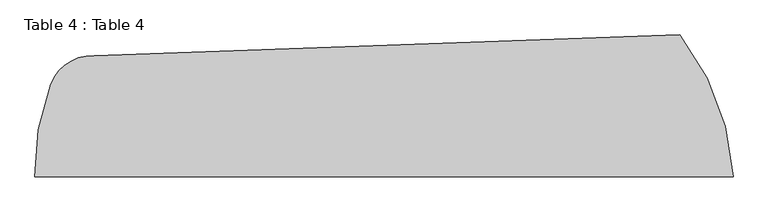
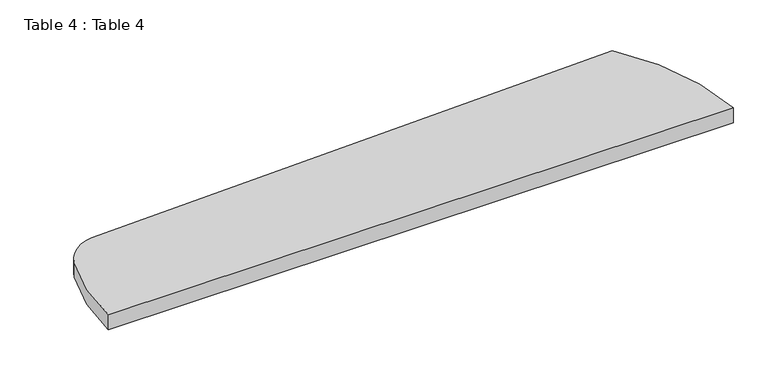
"""IFC4 building model written with IfcOpenShell, lengths in millimetres: furniture geometry, Table 4 : Table 4."""

from ifc_helpers import new_model, si_unit, point, frame, frame_2d, origin, place, context, project, spatial, polyline, circle_curve, trimmed, segment, composite_curve, outline, extrude, source, transform, mapped, element, save


def table_4_table_4_722f8e56(model_context):
    return source(origin(), model_context, "Body", "SweptSolid", [
        extrude(outline(composite_curve([segment(trimmed(circle_curve(frame_2d((1929.6173004, -6381.6325903)), 1451.9065758), [point((3077.0883729, -5492.0580613))], [point((3379.2077106, -6299.6548647))], False, "CARTESIAN"), True, "CONTINUOUS"), segment(polyline([(3379.2077106, -6299.6548647), (-589.7560586, -6299.6548647)]), True, "CONTINUOUS"), segment(trimmed(circle_curve(frame_2d((795.4843101, -6263.0932763)), 1385.7227821), [point((-589.7560586, -6299.6548647))], [point((-500.6672854, -5772.9721991))], False, "CARTESIAN"), True, "CONTINUOUS"), segment(trimmed(circle_curve(frame_2d((-266.8269365, -5861.3955626)), 250.0), [point((-500.6672854, -5772.9721991))], [point((-252.9313953, -5611.7820335))], False, "CARTESIAN"), True, "CONTINUOUS"), segment(trimmed(circle_curve(frame_2d((760.0219024, 12584.475549)), 18224.4304271), [point((-252.9313953, -5611.7820335))], [point((3077.0883729, -5492.0580613))], True, "CARTESIAN"), True, "CONTINUOUS")], self_intersect=False)), frame((0.0, 0.0, 800.0), z_axis=(0.0, 0.0, 1.0), x_axis=(1.0, 0.0, 0.0)), (0.0, 0.0, 1.0), 100.0),
    ])


if __name__ == "__main__":
    model = new_model("IFC4")
    model_context = context("Model", 3, world=origin())
    ifc_project = project(units=[si_unit("LENGTHUNIT", "METRE", prefix="MILLI")], contexts=[model_context])
    site = spatial("IfcSite", under=ifc_project)
    building = spatial("IfcBuilding", under=site)
    placement = place(None, origin())
    table_4_table_4_shape = table_4_table_4_722f8e56(model_context)
    element("IfcFurniture", 1, ObjectType="Table 4 : Table 4", at=placement, inside=building, context=model_context, shape_type="MappedRepresentation", body=[
        mapped(table_4_table_4_shape, transform((0.0, 0.0, 0.0), x_axis=(1.0, 0.0, 0.0), y_axis=(0.0, 1.0, 0.0), z_axis=(0.0, 0.0, 1.0))),
    ])
    save(model, "model.ifc")

# Revit data of these elements
# Type "Table 4 : Table 4"
#   COBie.Type.CreatedBy = "design@eagle.com"
#   COBie.Type.CreatedOn = "2016-09-13T05:47:35"
#   COBie.Type.Name = "Furniture_Table 4_Table 4"
#   COBie.Type.Category = "23-40 70 14 64 11 : Office Furniture"
#   COBie.Type.Description = ""
#   COBie.Type.Manufacturer = ""
#   COBie.Type.ModelNumber = ""
#   COBie.Type.ReplacementCost = 0
#   COBie.Type = yes
